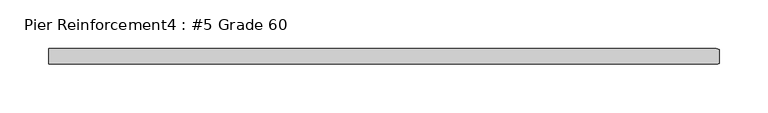
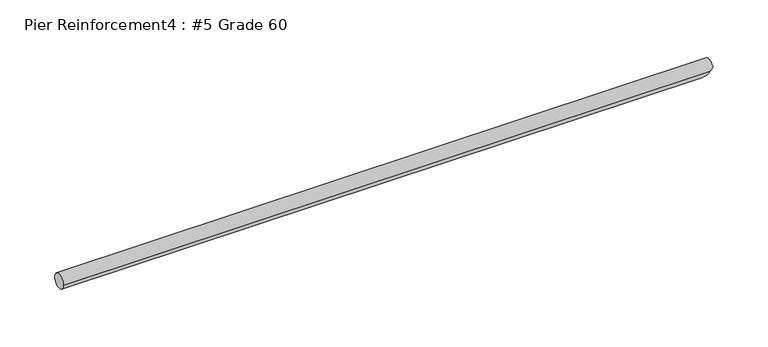
"""IFC4 building model written with IfcOpenShell, lengths in millimetres: proxy geometry, Pier Reinforcement4 : #5 Grade 60."""

from ifc_helpers import new_model, si_unit, frame, origin, place, context, project, spatial, circle_curve, ellipse_curve, source, transform, mapped, element, save
from ifc_brep_helpers import plane_surface, cylinder_surface, advanced_brep


def pier_reinforcement4_5_grade_60_3385e020(model_context):
    return source(origin(), model_context, "Body", "AdvancedBrep", [
        advanced_brep(
        [(590233.9922365, -534089.3915452, -52.3875), (590233.9922365, -534103.941223, -52.3875), (589548.1922365, -534088.7288841, -55.5625), (589548.1922365, -534104.6038841, -55.5625), (590230.8172365, -534104.6038841, -55.5625), (590230.8172365, -534088.7288841, -55.5625), (590222.8797365, -534096.6663841, -63.5)],
        [
            (0, 1, circle_curve(frame((590233.9922365, -534096.6663841, -55.5625), z_axis=(1.0, 0.0, 0.0), x_axis=(0.0, -1.0, 0.0)), 7.9375)),
            (1, 0),
            (2, 3, circle_curve(frame((589548.1922365, -534096.6663841, -55.5625), z_axis=(-1.0, 0.0, 0.0), x_axis=(0.0, -1.0, 0.0)), 7.9375)),
            (3, 2, circle_curve(frame((589548.1922365, -534096.6663841, -55.5625), z_axis=(-1.0, 0.0, 0.0), x_axis=(0.0, -1.0, 0.0)), 7.9375)),
            (3, 4),
            (4, 1, ellipse_curve(frame((590230.8172365, -534096.6663841, -55.5625), z_axis=(-0.7071067811865462, 0.0, 0.7071067811865489), x_axis=(0.7071067811865487, 0.0, 0.7071067811865462)), 11.2253202, 7.9375)),
            (0, 5, ellipse_curve(frame((590230.8172365, -534096.6663841, -55.5625), z_axis=(-0.7071067811865462, 0.0, 0.7071067811865489), x_axis=(0.7071067811865487, 0.0, 0.7071067811865462)), 11.2253202, 7.9375)),
            (5, 2),
            (5, 6, ellipse_curve(frame((590230.8172365, -534096.6663841, -55.5625), z_axis=(-0.7071067811865462, 0.0, 0.7071067811865489), x_axis=(0.7071067811865487, 0.0, 0.7071067811865462)), 11.2253202, 7.9375)),
            (6, 4, ellipse_curve(frame((590230.8172365, -534096.6663841, -55.5625), z_axis=(-0.7071067811865462, 0.0, 0.7071067811865489), x_axis=(0.7071067811865487, 0.0, 0.7071067811865462)), 11.2253202, 7.9375)),
        ],
        [
            plane_surface(frame((590233.9922365, -534104.6038841, -55.5625), z_axis=(1.0, 0.0, 0.0), x_axis=(0.0, 0.0, -1.0))),
            plane_surface(frame((589548.1922365, -534104.6038841, -55.5625), z_axis=(-1.0, 0.0, 0.0), x_axis=(0.0, 0.0, 1.0))),
            cylinder_surface(frame((589548.1922365, -534096.6663841, -55.5625), z_axis=(1.0, 0.0, 0.0), x_axis=(0.0, -1.0, 0.0)), 7.9375),
            plane_surface(frame((590222.8797365, -534128.4163841, -63.5), z_axis=(0.7071067811865462, 0.0, -0.7071067811865489), x_axis=(0.0, 1.0, 0.0))),
        ],
        [
            (0, [[1, 2]]),
            (1, [[3, 4]]),
            (2, [[-4, 5, 6, -1, 7, 8]]),
            (2, [[-3, -8, 9, 10, -5]]),
            (3, [[-2, -6, -10, -9, -7]]),
        ],
    ),
    ])


if __name__ == "__main__":
    model = new_model("IFC4")
    model_context = context("Model", 3, world=origin())
    ifc_project = project(units=[si_unit("LENGTHUNIT", "METRE", prefix="MILLI")], contexts=[model_context])
    site = spatial("IfcSite", under=ifc_project)
    building = spatial("IfcBuilding", under=site)
    placement = place(None, origin())
    pier_reinforcement4_5_grade_60_shape = pier_reinforcement4_5_grade_60_3385e020(model_context)
    element("IfcBuildingElementProxy", 1, Name="Pier Reinforcement4 : #5 Grade 60", ObjectType="Pier Reinforcement4 : #5 Grade 60", at=placement, inside=building, context=model_context, shape_type="MappedRepresentation", body=[
        mapped(pier_reinforcement4_5_grade_60_shape, transform((0.0, 0.0, 0.0), x_axis=(1.0, 0.0, 0.0), y_axis=(0.0, 1.0, 0.0), z_axis=(0.0, 0.0, 1.0))),
    ])
    save(model, "model.ifc")

# Revit data of these elements
# Element 1 (IfcBuildingElementProxy, "Pier Reinforcement4 : #5 Grade 60")
#   Materials on its faces: "#4 GR. 60 REINF. @ 16\" O.C. EW."
# Materials
#   "#4 GR. 60 REINF. @ 16\" O.C. EW.": class "Generic", colour RGB 84 83 81, transparency 0, Cost = 0
